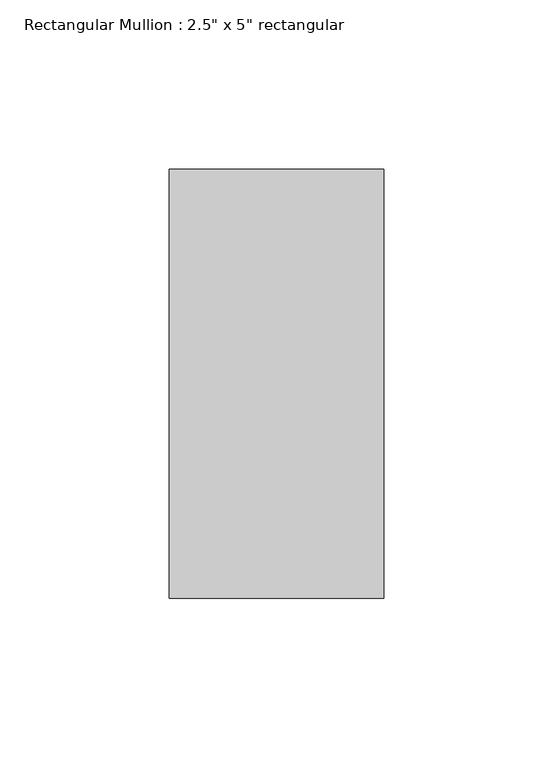
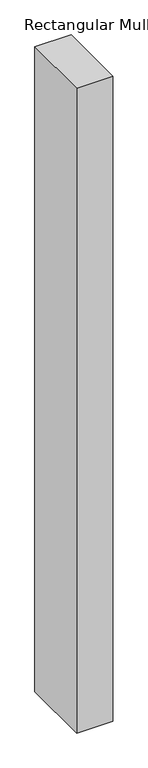
"""IFC4 building model written with IfcOpenShell, lengths in millimetres: member geometry."""

from ifc_helpers import new_model, si_unit, frame, origin, place, context, project, spatial, polyline, outline, extrude, source, transform, mapped, element, save


def member_c8b9ffd1(model_context):
    return source(origin(), model_context, "Body", "SweptSolid", [
        extrude(outline(polyline([(31.75, 63.5), (31.75, -63.5), (-31.75, -63.5), (-31.75, 63.5), (31.75, 63.5)])), frame((0.0, 0.0, -1198.0333333), z_axis=(0.0, 0.0, 1.0), x_axis=(1.0, 0.0, 0.0)), (0.0, 0.0, 1.0), 1198.0333333),
    ])


if __name__ == "__main__":
    model = new_model("IFC4")
    model_context = context("Model", 3, world=origin())
    ifc_project = project(units=[si_unit("LENGTHUNIT", "METRE", prefix="MILLI")], contexts=[model_context])
    site = spatial("IfcSite", under=ifc_project)
    building = spatial("IfcBuilding", under=site)
    placement = place(None, origin())
    member_shape = member_c8b9ffd1(model_context)
    element("IfcMember", 1, ObjectType="Rectangular Mullion : 2.5\" x 5\" rectangular", at=placement, inside=building, context=model_context, shape_type="MappedRepresentation", body=[
        mapped(member_shape, transform((0.0, 0.0, 0.0), x_axis=(1.0, 0.0, 0.0), y_axis=(0.0, 1.0, 0.0), z_axis=(0.0, 0.0, 1.0))),
    ])
    save(model, "model.ifc")

# Revit data of these elements
# Type "Rectangular Mullion : 2.5\" x 5\" rectangular"
#   built-in parameter 1007304 = 0.416667 (stored number, unit not read)
#   built-in parameter 1007301 = 0.104167 (stored number, unit not read)
#   built-in parameter 1007300 = 0.104167 (stored number, unit not read)
